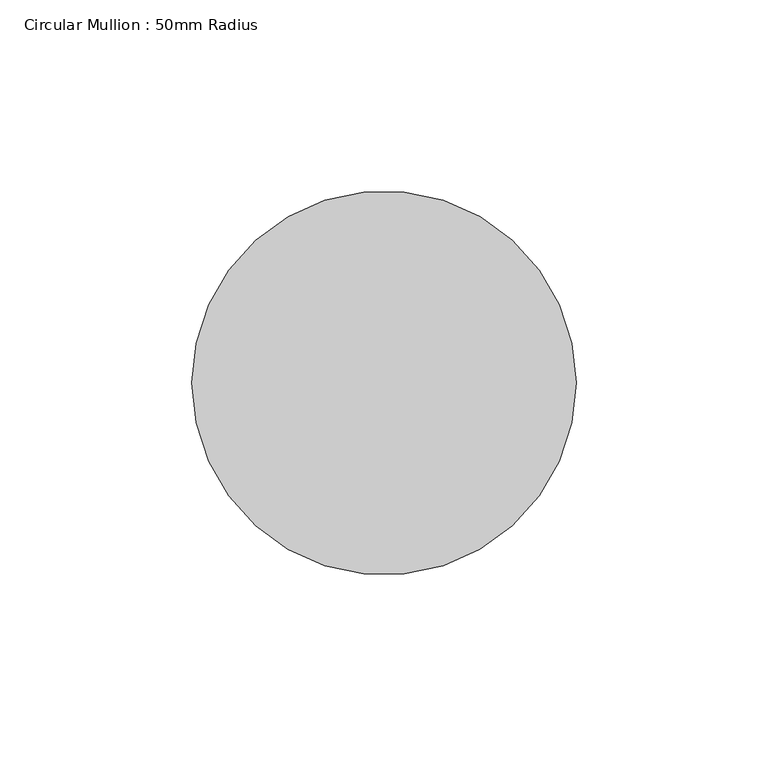
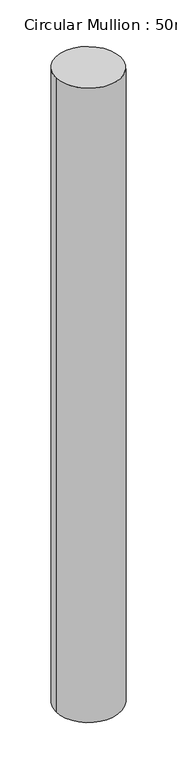
"""IFC4 building model written with IfcOpenShell, lengths in millimetres: member geometry, Circular Mullion : 50mm Radius."""

from ifc_helpers import new_model, si_unit, frame, origin, place, context, project, spatial, ellipse_curve, source, transform, mapped, element, save
from ifc_brep_helpers import plane_surface, cylinder_surface, advanced_brep


def circular_mullion_50mm_radius_4f7f5064(model_context):
    return source(origin(), model_context, "Body", "AdvancedBrep", [
        advanced_brep(
        [(-100.0, 0.0, 1.4865198), (0.0, 0.0, 0.0), (0.0, 0.0, -1029.1375724), (-100.0, 0.0, -1030.5891417)],
        [
            (0, 1, ellipse_curve(frame((-50.0, 0.0, 0.7432599), z_axis=(-0.01486192144897568, -0.014831316262930869, -0.9997795533760199), x_axis=(-0.7076791889830483, -0.706221863743292, 0.020996300894346814)), 50.0110248, 50.0)),
            (1, 2),
            (2, 3, ellipse_curve(frame((-50.0, 0.0, -1029.8633571), z_axis=(-0.014512641812093979, -0.014482755898340085, 0.9997897944114168), x_axis=(0.7076864379486502, 0.7062290977811482, 0.020502853235022895)), 50.0105125, 50.0)),
            (3, 0),
            (1, 0, ellipse_curve(frame((-50.0, 0.0, 0.7432599), z_axis=(-0.01486192144897568, -0.014831316262930869, -0.9997795533760199), x_axis=(-0.7076791889830483, -0.706221863743292, 0.020996300894346814)), 50.0110248, 50.0)),
            (3, 2, ellipse_curve(frame((-50.0, 0.0, -1029.8633571), z_axis=(-0.014512641812093979, -0.014482755898340085, 0.9997897944114168), x_axis=(0.7076864379486502, 0.7062290977811482, 0.020502853235022895)), 50.0105125, 50.0)),
        ],
        [
            cylinder_surface(frame((-50.0, 0.0, 0.0), z_axis=(0.0, 0.0, 1.0), x_axis=(1.0, 0.0, 0.0)), 50.0),
            plane_surface(frame((-215.3038871, 215.7481778, 0.0), z_axis=(0.01486192144897568, 0.014831316262930869, 0.9997795533760199), x_axis=(0.707679188983048, 0.706221863743292, -0.020996300894362344))),
            plane_surface(frame((-215.3038871, 215.7481778, -1029.1375724), z_axis=(0.014512641812093982, 0.014482755898340088, -0.999789794411417), x_axis=(0.7076864379486502, 0.7062290977811482, 0.020502853235026656))),
        ],
        [
            (0, [[1, 2, 3, 4]]),
            (0, [[5, -4, 6, -2]]),
            (1, [[-1, -5]]),
            (2, [[-6, -3]]),
        ],
    ),
    ])


if __name__ == "__main__":
    model = new_model("IFC4")
    model_context = context("Model", 3, world=origin())
    ifc_project = project(units=[si_unit("LENGTHUNIT", "METRE", prefix="MILLI")], contexts=[model_context])
    site = spatial("IfcSite", under=ifc_project)
    building = spatial("IfcBuilding", under=site)
    placement = place(None, origin())
    circular_mullion_50mm_radius_shape = circular_mullion_50mm_radius_4f7f5064(model_context)
    element("IfcMember", 1, ObjectType="Circular Mullion : 50mm Radius", at=placement, inside=building, context=model_context, shape_type="MappedRepresentation", body=[
        mapped(circular_mullion_50mm_radius_shape, transform((0.0, 0.0, 0.0), x_axis=(1.0, 0.0, 0.0), y_axis=(0.0, 1.0, 0.0), z_axis=(0.0, 0.0, 1.0))),
    ])
    save(model, "model.ifc")

# Revit data of these elements
# Type "Circular Mullion : 50mm Radius"
#   built-in parameter 1007350 = 0.164042 (stored number, unit not read)
# Element 1 (IfcMember, "Circular Mullion : 50mm Radius")
#   Materials on its faces: "Aluminium"
# Materials
#   "Aluminium": class "Metal", colour RGB 247 247 247, transparency 0, Description = "Aluminium 6061", Cost = 0
